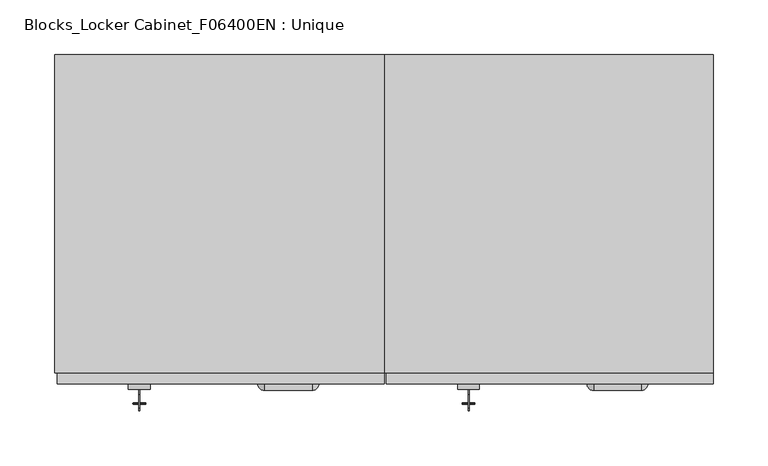
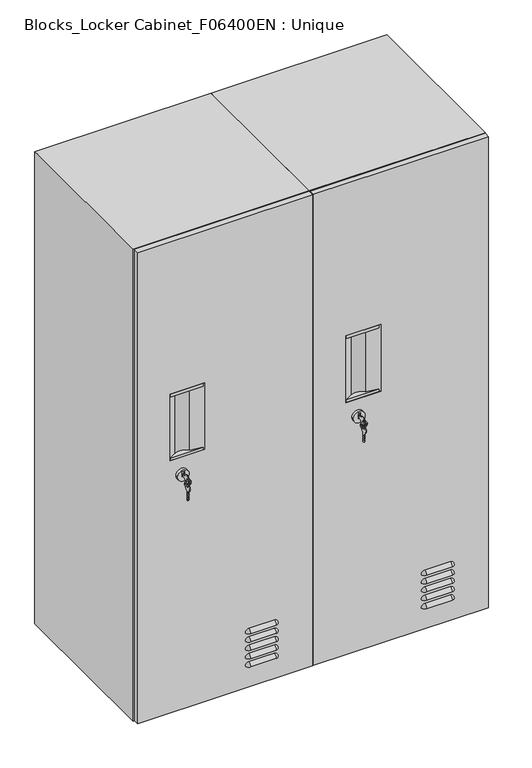
"""IFC4 building model written with IfcOpenShell, lengths in millimetres: furniture geometry, Blocks_Locker Cabinet_F06400EN : Unique."""

from ifc_helpers import new_model, si_unit, point, frame, frame_2d, origin, place, context, project, spatial, polyline, circle_curve, ellipse_curve, trimmed, segment, composite_curve, outline, extrude, faceted_brep, source, transform, mapped, element, save
from ifc_brep_helpers import plane_surface, cylinder_surface, revolved_surface, advanced_brep


def blocks_locker_cabinet_f06400en_unique_ebf76149(model_context):
    return source(origin(), model_context, "Body", "SolidModel", [
        advanced_brep(
        [(-83.0, -12.5, 1375.0), (-63.0, -12.5, 1375.0), (-71.1588195, -12.5, 1382.0962926), (-71.1588195, -12.5, 1372.8618188), (-74.8411805, -12.5, 1372.8618188), (-74.8411805, -12.5, 1382.0962926), (-83.0, -7.5, 1375.0), (-63.0, -7.5, 1375.0), (-83.0, -10.7450625, 1375.0), (-63.0, -10.7450625, 1375.0), (-71.1588195, -10.7450625, 1382.0962926), (-71.1588195, -10.7450625, 1372.8618188), (-74.8411805, -10.7450625, 1372.8618188), (-74.8411805, -10.7450625, 1382.0962926)],
        [
            (0, 1, circle_curve(frame((-73.0, -12.5, 1375.0), z_axis=(0.0, -1.0, 0.0), x_axis=(1.0, 0.0, 0.0)), 10.0)),
            (1, 0, circle_curve(frame((-73.0, -12.5, 1375.0), z_axis=(0.0, -1.0, 0.0), x_axis=(1.0, 0.0, 0.0)), 10.0)),
            (2, 3),
            (3, 4),
            (4, 5),
            (5, 2),
            (6, 7, circle_curve(frame((-73.0, -7.5, 1375.0), z_axis=(0.0, 1.0, 0.0), x_axis=(1.0, 0.0, 0.0)), 10.0)),
            (7, 6, circle_curve(frame((-73.0, -7.5, 1375.0), z_axis=(0.0, 1.0, 0.0), x_axis=(1.0, 0.0, 0.0)), 10.0)),
            (0, 8),
            (8, 6),
            (7, 9),
            (9, 1),
            (2, 10),
            (10, 11),
            (11, 3),
            (11, 12),
            (12, 4),
            (12, 13),
            (13, 5),
            (13, 10),
        ],
        [
            plane_surface(frame((-63.0, -12.5, 1375.0), z_axis=(0.0, -1.0, 0.0), x_axis=(0.0, 0.0, 1.0))),
            plane_surface(frame((-63.0, -7.5, 1375.0), z_axis=(0.0, 1.0, 0.0), x_axis=(0.0, 0.0, -1.0))),
            cylinder_surface(frame((-73.0, -7.5, 1375.0), z_axis=(0.0, -1.0, 0.0), x_axis=(1.0, 0.0, 0.0)), 10.0),
            plane_surface(frame((-71.1588195, -12.5, 1382.0962926), z_axis=(-1.0, 0.0, 0.0), x_axis=(0.0, 1.0, 0.0))),
            plane_surface(frame((-71.1588195, -12.5, 1372.8618188), z_axis=(0.0, 0.0, 1.0), x_axis=(0.0, 1.0, 0.0))),
            plane_surface(frame((-74.8411805, -12.5, 1372.8618188), z_axis=(1.0, 0.0, 0.0), x_axis=(0.0, 1.0, 0.0))),
            plane_surface(frame((-74.8411805, -12.5, 1382.0962926), z_axis=(0.0, 0.0, -1.0), x_axis=(0.0, 1.0, 0.0))),
            plane_surface(frame((-63.0, -10.7450625, 1375.0), z_axis=(0.0, -1.0, 0.0), x_axis=(0.0, 0.0, 1.0))),
        ],
        [
            (0, [[1, 2], [3, 4, 5, 6]]),
            (1, [[7, 8]]),
            (2, [[-1, 9, 10, -8, 11, 12]]),
            (2, [[-2, -12, -11, -7, -10, -9]]),
            (3, [[-3, 13, 14, 15]]),
            (4, [[-4, -15, 16, 17]]),
            (5, [[-5, -17, 18, 19]]),
            (6, [[-6, -19, 20, -13]]),
            (7, [[-14, -20, -18, -16]]),
        ],
    ),
        extrude(outline(composite_curve([segment(trimmed(circle_curve(frame_2d((-23.0067332, 1375.0)), 6.5414185), [point((-16.8246351, 1372.8618188))], [point((-17.0336838, 1377.6669902))], False, "CARTESIAN"), True, "CONTINUOUS"), segment(polyline([(-17.0336838, 1377.6669902), (-10.7450625, 1377.6669902), (-10.7450625, 1372.8618188), (-12.0321832, 1372.8618188)]), True, "CONTINUOUS"), segment(trimmed(circle_curve(frame_2d((-12.908516, 1372.8618188)), 0.8763328), [point((-12.0321832, 1372.8618188))], [point((-13.7848488, 1372.8618188))], True, "CARTESIAN"), True, "CONTINUOUS"), segment(polyline([(-13.7848488, 1372.8618188), (-16.8246351, 1372.8618188)]), True, "CONTINUOUS")], self_intersect=False), holes=[composite_curve([segment(trimmed(circle_curve(frame_2d((-25.6281997, 1375.0)), 1.688217), [point((-27.3164167, 1375.0))], [point((-23.9399827, 1375.0))], True, "CARTESIAN"), True, "CONTINUOUS"), segment(trimmed(circle_curve(frame_2d((-25.6281997, 1375.0)), 1.688217), [point((-23.9399827, 1375.0))], [point((-27.3164167, 1375.0))], True, "CARTESIAN"), True, "CONTINUOUS")], self_intersect=False)]), frame((-73.4043078, 0.0, 0.0), z_axis=(1.0, 0.0, 0.0), x_axis=(0.0, 1.0, 0.0)), (0.0, 0.0, 1.0), 0.9157402),
        extrude(outline(composite_curve([segment(trimmed(circle_curve(frame_2d((-25.6743188, 1360.9839856)), 6.5414185), [point((-27.8125, 1354.8018875))], [point((-24.2573286, 1354.5978839))], False, "CARTESIAN"), True, "CONTINUOUS"), segment(polyline([(-24.2573286, 1354.5978839), (-24.2573286, 1337.7095301), (-25.9613419, 1337.7095301), (-27.8125, 1340.3532579), (-27.8125, 1342.0094356)]), True, "CONTINUOUS"), segment(trimmed(circle_curve(frame_2d((-27.8125, 1342.8857684)), 0.8763328), [point((-27.8125, 1342.0094356))], [point((-27.8125, 1343.7621012))], True, "CARTESIAN"), True, "CONTINUOUS"), segment(polyline([(-27.8125, 1343.7621012), (-27.8125, 1346.0094356)]), True, "CONTINUOUS"), segment(trimmed(circle_curve(frame_2d((-27.8125, 1346.8857684)), 0.8763328), [point((-27.8125, 1346.0094356))], [point((-27.8125, 1347.7621012))], True, "CARTESIAN"), True, "CONTINUOUS"), segment(polyline([(-27.8125, 1347.7621012), (-27.8125, 1350.0094356)]), True, "CONTINUOUS"), segment(trimmed(circle_curve(frame_2d((-27.8125, 1350.8857684)), 0.8763328), [point((-27.8125, 1350.0094356))], [point((-27.8125, 1351.7621012))], True, "CARTESIAN"), True, "CONTINUOUS"), segment(polyline([(-27.8125, 1351.7621012), (-27.8125, 1354.8018875)]), True, "CONTINUOUS")], self_intersect=False), holes=[composite_curve([segment(trimmed(circle_curve(frame_2d((-25.6743188, 1363.6054521)), 1.688217), [point((-25.6743188, 1365.2936691))], [point((-25.6743188, 1361.9172351))], True, "CARTESIAN"), True, "CONTINUOUS"), segment(trimmed(circle_curve(frame_2d((-25.6743188, 1363.6054521)), 1.688217), [point((-25.6743188, 1361.9172351))], [point((-25.6743188, 1365.2936691))], True, "CARTESIAN"), True, "CONTINUOUS")], self_intersect=False)]), frame((-73.4043078, 0.0, 0.0), z_axis=(1.0, 0.0, 0.0), x_axis=(0.0, 1.0, 0.0)), (0.0, 0.0, 1.0), 0.9157402),
        advanced_brep(
        [(-68.8, -25.663019, 1369.4000012), (-77.2, -25.663019, 1369.4000012), (-78.8, -25.663019, 1369.4000012), (-67.2, -25.663019, 1369.4000012)],
        [
            (0, 1, circle_curve(frame((-73.0, -25.663019, 1369.4000012), z_axis=(0.0, 1.0, 0.0), x_axis=(-1.0, 0.0, 0.0)), 4.2)),
            (1, 2, circle_curve(frame((-78.0, -25.663019, 1369.4000012), z_axis=(0.0, 0.0, -1.0), x_axis=(1.0, 0.0, 0.0)), 0.8)),
            (2, 3, circle_curve(frame((-73.0, -25.663019, 1369.4000012), z_axis=(0.0, -1.0, 0.0), x_axis=(-1.0, 0.0, 0.0)), 5.8)),
            (3, 0, circle_curve(frame((-68.0, -25.663019, 1369.4000012), z_axis=(0.0, 0.0, -1.0), x_axis=(-1.0, 0.0, 0.0)), 0.8)),
            (2, 1, circle_curve(frame((-78.0, -25.663019, 1369.4000012), z_axis=(0.0, 0.0, -1.0), x_axis=(1.0, 0.0, 0.0)), 0.8)),
            (0, 3, circle_curve(frame((-68.0, -25.663019, 1369.4000012), z_axis=(0.0, 0.0, -1.0), x_axis=(-1.0, 0.0, 0.0)), 0.8)),
            (1, 0, circle_curve(frame((-73.0, -25.663019, 1369.4000012), z_axis=(0.0, 1.0, 0.0), x_axis=(1.0, 0.0, 0.0)), 4.2)),
            (3, 2, circle_curve(frame((-73.0, -25.663019, 1369.4000012), z_axis=(0.0, -1.0, 0.0), x_axis=(1.0, 0.0, 0.0)), 5.8)),
        ],
        [
            revolved_surface(trimmed(ellipse_curve(frame((-78.0, -25.663019, 1369.4000012), z_axis=(0.0, 0.0, 1.0), x_axis=(1.0, 0.0, 0.0)), 0.8, 0.8), [point((-78.8, -25.663019, 1369.4000012))], [point((-77.2, -25.663019, 1369.4000012))], True, "CARTESIAN"), (-73.0, 2.5, 1369.4000012), (0.0, -1.0, 0.0)),
            revolved_surface(trimmed(ellipse_curve(frame((-78.0, -25.663019, 1369.4000012), z_axis=(0.0, 0.0, 1.0), x_axis=(1.0, 0.0, 0.0)), 0.8, 0.8), [point((-77.2, -25.663019, 1369.4000012))], [point((-78.8, -25.663019, 1369.4000012))], True, "CARTESIAN"), (-73.0, 2.5, 1369.4000012), (0.0, -1.0, 0.0)),
            revolved_surface(trimmed(ellipse_curve(frame((-68.0, -25.663019, 1369.4000012), z_axis=(0.0, 0.0, -1.0), x_axis=(-1.0, 0.0, 0.0)), 0.8, 0.8), [point((-67.2, -25.663019, 1369.4000012))], [point((-68.8, -25.663019, 1369.4000012))], True, "CARTESIAN"), (-73.0, 2.5, 1369.4000012), (0.0, -1.0, 0.0)),
            revolved_surface(trimmed(ellipse_curve(frame((-68.0, -25.663019, 1369.4000012), z_axis=(0.0, 0.0, -1.0), x_axis=(-1.0, 0.0, 0.0)), 0.8, 0.8), [point((-68.8, -25.663019, 1369.4000012))], [point((-67.2, -25.663019, 1369.4000012))], True, "CARTESIAN"), (-73.0, 2.5, 1369.4000012), (0.0, -1.0, 0.0)),
        ],
        [
            (0, [[1, 2, 3, 4]]),
            (1, [[-3, 5, -1, 6]]),
            (2, [[7, -4, 8, -2]]),
            (3, [[-8, -6, -7, -5]]),
        ],
    ),
        advanced_brep(
        [(-148.0, -7.5, 1799.0), (150.0, -7.5, 1799.0), (150.0, 2.5, 1799.0), (-148.0, 2.5, 1799.0), (-148.0, -7.5, 951.0), (-148.0, 2.5, 951.0), (150.0, 2.5, 951.0), (150.0, -7.5, 951.0), (-93.0, -7.5, 1525.0), (-33.7890736, -7.5, 1525.0), (-33.7890736, -7.5, 1405.0), (-93.0, -7.5, 1405.0), (-80.6526901, -0.3712773, 1525.0), (-57.2105549, -3.975278, 1525.0), (-80.6526901, -0.3712773, 1405.0), (-57.2105549, -3.975278, 1405.0)],
        [
            (0, 1),
            (1, 2),
            (2, 3),
            (3, 0),
            (4, 5),
            (5, 6),
            (6, 7),
            (7, 4),
            (0, 4),
            (7, 1),
            (8, 9),
            (9, 10),
            (10, 11),
            (11, 8),
            (6, 2),
            (5, 3),
            (12, 13, circle_curve(frame((-71.1776523, -16.7825242, 1525.0), z_axis=(0.0, 0.0, -1.0), x_axis=(0.0, -1.0, 0.0)), 18.9500756)),
            (13, 9),
            (8, 12),
            (14, 11),
            (10, 15),
            (15, 14, circle_curve(frame((-71.1776523, -16.7825242, 1405.0), z_axis=(0.0, 0.0, 1.0), x_axis=(0.0, -1.0, 0.0)), 18.9500756)),
            (14, 12),
            (13, 15),
        ],
        [
            plane_surface(frame((150.0, -7.5, 1799.0), z_axis=(0.0, 0.0, 1.0), x_axis=(1.0, 0.0, 0.0))),
            plane_surface(frame((150.0, -7.5, 951.0), z_axis=(0.0, 0.0, -1.0), x_axis=(-1.0, 0.0, 0.0))),
            plane_surface(frame((-148.0, -7.5, 1799.0), z_axis=(0.0, -1.0, 0.0), x_axis=(0.0, 0.0, -1.0))),
            plane_surface(frame((150.0, -7.5, 1799.0), z_axis=(1.0, 0.0, 0.0), x_axis=(0.0, 0.0, -1.0))),
            plane_surface(frame((150.0, 2.5, 1799.0), z_axis=(0.0, 1.0, 0.0), x_axis=(0.0, 0.0, -1.0))),
            plane_surface(frame((-148.0, 2.5, 1799.0), z_axis=(-1.0, 0.0, 0.0), x_axis=(0.0, 0.0, -1.0))),
            plane_surface(frame((-93.0, -7.5, 1525.0), z_axis=(0.0, 0.0, -1.0), x_axis=(-0.866025403784437, -0.5000000000000028, 0.0))),
            plane_surface(frame((-93.0, -7.5, 1405.0), z_axis=(0.0, 0.0, 1.0), x_axis=(0.866025403784437, 0.5000000000000028, 0.0))),
            plane_surface(frame((-80.6526901, -0.3712773, 1525.0), z_axis=(0.5000000000000028, -0.866025403784437, 0.0), x_axis=(0.0, 0.0, -1.0))),
            plane_surface(frame((-33.7890736, -7.5, 1525.0), z_axis=(-0.14881527984319862, -0.9888650122666847, 0.0), x_axis=(0.0, 0.0, -1.0))),
            revolved_surface(polyline([(-71.1776523, -35.7325998, 1525.0), (-71.1776523, -35.7325998, 1405.0)]), (-71.1776523, -16.7825242, 1405.0), (0.0, 0.0, 1.0)),
        ],
        [
            (0, [[1, 2, 3, 4]]),
            (1, [[5, 6, 7, 8]]),
            (2, [[-1, 9, -8, 10], [11, 12, 13, 14]]),
            (3, [[-2, -10, -7, 15]]),
            (4, [[-3, -15, -6, 16]]),
            (5, [[-4, -16, -5, -9]]),
            (6, [[17, 18, -11, 19]]),
            (7, [[20, -13, 21, 22]]),
            (8, [[-19, -14, -20, 23]]),
            (9, [[-18, 24, -21, -12]]),
            (10, [[-17, -23, -22, -24]]),
        ],
    ),
        advanced_brep(
        [(35.0, -7.5, 991.0), (41.0, -7.5, 997.0), (84.5189667, -7.5, 997.0), (90.5189667, -7.5, 991.0), (84.5189667, -13.5, 991.0), (41.0, -13.5, 991.0)],
        [
            (0, 1, circle_curve(frame((41.0, -7.5, 991.0), z_axis=(0.0, 1.0, 0.0), x_axis=(1.0, 0.0, 0.0)), 6.0)),
            (1, 2),
            (2, 3, circle_curve(frame((84.5189667, -7.5, 991.0), z_axis=(0.0, 1.0, 0.0), x_axis=(1.0, 0.0, 0.0)), 6.0)),
            (3, 0),
            (3, 4, circle_curve(frame((84.5189667, -7.5, 991.0), z_axis=(0.0, 0.0, -1.0), x_axis=(1.0, 0.0, 0.0)), 6.0)),
            (4, 5),
            (5, 0, circle_curve(frame((41.0, -7.5, 991.0), z_axis=(0.0, 0.0, -1.0), x_axis=(1.0, 0.0, 0.0)), 6.0)),
            (5, 1, circle_curve(frame((41.0, -7.5, 991.0), z_axis=(-1.0, 0.0, 0.0), x_axis=(0.0, 0.0, 1.0)), 6.0)),
            (4, 2, circle_curve(frame((84.5189667, -7.5, 991.0), z_axis=(-1.0, 0.0, 0.0), x_axis=(0.0, 0.0, 1.0)), 6.0)),
        ],
        [
            plane_surface(frame((85.0, -7.5, 991.0), z_axis=(0.0, 1.0, 0.0), x_axis=(0.0, 0.0, 1.0))),
            plane_surface(frame((85.0, -7.5, 991.0), z_axis=(0.0, 0.0, -1.0), x_axis=(0.0, -1.0, 0.0))),
            revolved_surface(trimmed(ellipse_curve(frame((41.0, -7.5, 991.0), z_axis=(0.0, 1.0, 0.0), x_axis=(1.0, 0.0, 0.0)), 6.0, 6.0), [point((35.0, -7.5, 991.0))], [point((41.0, -7.5, 997.0))], True, "CARTESIAN"), (85.0, -7.5, 991.0), (1.0, 0.0, 0.0)),
            cylinder_surface(frame((85.0, -7.5, 991.0), z_axis=(1.0, 0.0, 0.0), x_axis=(0.0, 0.0, 1.0)), 6.0),
            revolved_surface(trimmed(ellipse_curve(frame((84.5189667, -7.5, 991.0), z_axis=(0.0, 1.0, 0.0), x_axis=(1.0, 0.0, 0.0)), 6.0, 6.0), [point((84.5189667, -7.5, 997.0))], [point((90.5189667, -7.5, 991.0))], True, "CARTESIAN"), (85.0, -7.5, 991.0), (1.0, 0.0, 0.0)),
        ],
        [
            (0, [[1, 2, 3, 4]]),
            (1, [[5, 6, 7, -4]]),
            (2, [[8, -1, -7]]),
            (3, [[9, -2, -8, -6]]),
            (4, [[-3, -9, -5]]),
        ],
    ),
        advanced_brep(
        [(35.0, -7.5, 1006.0), (41.0, -7.5, 1012.0), (84.5189667, -7.5, 1012.0), (90.5189667, -7.5, 1006.0), (84.5189667, -13.5, 1006.0), (41.0, -13.5, 1006.0)],
        [
            (0, 1, circle_curve(frame((41.0, -7.5, 1006.0), z_axis=(0.0, 1.0, 0.0), x_axis=(1.0, 0.0, 0.0)), 6.0)),
            (1, 2),
            (2, 3, circle_curve(frame((84.5189667, -7.5, 1006.0), z_axis=(0.0, 1.0, 0.0), x_axis=(1.0, 0.0, 0.0)), 6.0)),
            (3, 0),
            (3, 4, circle_curve(frame((84.5189667, -7.5, 1006.0), z_axis=(0.0, 0.0, -1.0), x_axis=(1.0, 0.0, 0.0)), 6.0)),
            (4, 5),
            (5, 0, circle_curve(frame((41.0, -7.5, 1006.0), z_axis=(0.0, 0.0, -1.0), x_axis=(1.0, 0.0, 0.0)), 6.0)),
            (5, 1, circle_curve(frame((41.0, -7.5, 1006.0), z_axis=(-1.0, 0.0, 0.0), x_axis=(0.0, 0.0, 1.0)), 6.0)),
            (4, 2, circle_curve(frame((84.5189667, -7.5, 1006.0), z_axis=(-1.0, 0.0, 0.0), x_axis=(0.0, 0.0, 1.0)), 6.0)),
        ],
        [
            plane_surface(frame((85.0, -7.5, 1006.0), z_axis=(0.0, 1.0, 0.0), x_axis=(0.0, 0.0, 1.0))),
            plane_surface(frame((85.0, -7.5, 1006.0), z_axis=(0.0, 0.0, -1.0), x_axis=(0.0, -1.0, 0.0))),
            revolved_surface(trimmed(ellipse_curve(frame((41.0, -7.5, 1006.0), z_axis=(0.0, 1.0, 0.0), x_axis=(1.0, 0.0, 0.0)), 6.0, 6.0), [point((35.0, -7.5, 1006.0))], [point((41.0, -7.5, 1012.0))], True, "CARTESIAN"), (85.0, -7.5, 1006.0), (1.0, 0.0, 0.0)),
            cylinder_surface(frame((85.0, -7.5, 1006.0), z_axis=(1.0, 0.0, 0.0), x_axis=(0.0, 0.0, 1.0)), 6.0),
            revolved_surface(trimmed(ellipse_curve(frame((84.5189667, -7.5, 1006.0), z_axis=(0.0, 1.0, 0.0), x_axis=(1.0, 0.0, 0.0)), 6.0, 6.0), [point((84.5189667, -7.5, 1012.0))], [point((90.5189667, -7.5, 1006.0))], True, "CARTESIAN"), (85.0, -7.5, 1006.0), (1.0, 0.0, 0.0)),
        ],
        [
            (0, [[1, 2, 3, 4]]),
            (1, [[5, 6, 7, -4]]),
            (2, [[8, -1, -7]]),
            (3, [[9, -2, -8, -6]]),
            (4, [[-3, -9, -5]]),
        ],
    ),
        advanced_brep(
        [(35.0, -7.5, 1021.0), (41.0, -7.5, 1027.0), (84.5189667, -7.5, 1027.0), (90.5189667, -7.5, 1021.0), (84.5189667, -13.5, 1021.0), (41.0, -13.5, 1021.0)],
        [
            (0, 1, circle_curve(frame((41.0, -7.5, 1021.0), z_axis=(0.0, 1.0, 0.0), x_axis=(1.0, 0.0, 0.0)), 6.0)),
            (1, 2),
            (2, 3, circle_curve(frame((84.5189667, -7.5, 1021.0), z_axis=(0.0, 1.0, 0.0), x_axis=(1.0, 0.0, 0.0)), 6.0)),
            (3, 0),
            (3, 4, circle_curve(frame((84.5189667, -7.5, 1021.0), z_axis=(0.0, 0.0, -1.0), x_axis=(1.0, 0.0, 0.0)), 6.0)),
            (4, 5),
            (5, 0, circle_curve(frame((41.0, -7.5, 1021.0), z_axis=(0.0, 0.0, -1.0), x_axis=(1.0, 0.0, 0.0)), 6.0)),
            (5, 1, circle_curve(frame((41.0, -7.5, 1021.0), z_axis=(-1.0, 0.0, 0.0), x_axis=(0.0, 0.0, 1.0)), 6.0)),
            (4, 2, circle_curve(frame((84.5189667, -7.5, 1021.0), z_axis=(-1.0, 0.0, 0.0), x_axis=(0.0, 0.0, 1.0)), 6.0)),
        ],
        [
            plane_surface(frame((85.0, -7.5, 1021.0), z_axis=(0.0, 1.0, 0.0), x_axis=(0.0, 0.0, 1.0))),
            plane_surface(frame((85.0, -7.5, 1021.0), z_axis=(0.0, 0.0, -1.0), x_axis=(0.0, -1.0, 0.0))),
            revolved_surface(trimmed(ellipse_curve(frame((41.0, -7.5, 1021.0), z_axis=(0.0, 1.0, 0.0), x_axis=(1.0, 0.0, 0.0)), 6.0, 6.0), [point((35.0, -7.5, 1021.0))], [point((41.0, -7.5, 1027.0))], True, "CARTESIAN"), (85.0, -7.5, 1021.0), (1.0, 0.0, 0.0)),
            cylinder_surface(frame((85.0, -7.5, 1021.0), z_axis=(1.0, 0.0, 0.0), x_axis=(0.0, 0.0, 1.0)), 6.0),
            revolved_surface(trimmed(ellipse_curve(frame((84.5189667, -7.5, 1021.0), z_axis=(0.0, 1.0, 0.0), x_axis=(1.0, 0.0, 0.0)), 6.0, 6.0), [point((84.5189667, -7.5, 1027.0))], [point((90.5189667, -7.5, 1021.0))], True, "CARTESIAN"), (85.0, -7.5, 1021.0), (1.0, 0.0, 0.0)),
        ],
        [
            (0, [[1, 2, 3, 4]]),
            (1, [[5, 6, 7, -4]]),
            (2, [[8, -1, -7]]),
            (3, [[9, -2, -8, -6]]),
            (4, [[-3, -9, -5]]),
        ],
    ),
        advanced_brep(
        [(35.0, -7.5, 1036.0), (41.0, -7.5, 1042.0), (84.5189667, -7.5, 1042.0), (90.5189667, -7.5, 1036.0), (84.5189667, -13.5, 1036.0), (41.0, -13.5, 1036.0)],
        [
            (0, 1, circle_curve(frame((41.0, -7.5, 1036.0), z_axis=(0.0, 1.0, 0.0), x_axis=(1.0, 0.0, 0.0)), 6.0)),
            (1, 2),
            (2, 3, circle_curve(frame((84.5189667, -7.5, 1036.0), z_axis=(0.0, 1.0, 0.0), x_axis=(1.0, 0.0, 0.0)), 6.0)),
            (3, 0),
            (3, 4, circle_curve(frame((84.5189667, -7.5, 1036.0), z_axis=(0.0, 0.0, -1.0), x_axis=(1.0, 0.0, 0.0)), 6.0)),
            (4, 5),
            (5, 0, circle_curve(frame((41.0, -7.5, 1036.0), z_axis=(0.0, 0.0, -1.0), x_axis=(1.0, 0.0, 0.0)), 6.0)),
            (5, 1, circle_curve(frame((41.0, -7.5, 1036.0), z_axis=(-1.0, 0.0, 0.0), x_axis=(0.0, 0.0, 1.0)), 6.0)),
            (4, 2, circle_curve(frame((84.5189667, -7.5, 1036.0), z_axis=(-1.0, 0.0, 0.0), x_axis=(0.0, 0.0, 1.0)), 6.0)),
        ],
        [
            plane_surface(frame((85.0, -7.5, 1036.0), z_axis=(0.0, 1.0, 0.0), x_axis=(0.0, 0.0, 1.0))),
            plane_surface(frame((85.0, -7.5, 1036.0), z_axis=(0.0, 0.0, -1.0), x_axis=(0.0, -1.0, 0.0))),
            revolved_surface(trimmed(ellipse_curve(frame((41.0, -7.5, 1036.0), z_axis=(0.0, 1.0, 0.0), x_axis=(1.0, 0.0, 0.0)), 6.0, 6.0), [point((35.0, -7.5, 1036.0))], [point((41.0, -7.5, 1042.0))], True, "CARTESIAN"), (85.0, -7.5, 1036.0), (1.0, 0.0, 0.0)),
            cylinder_surface(frame((85.0, -7.5, 1036.0), z_axis=(1.0, 0.0, 0.0), x_axis=(0.0, 0.0, 1.0)), 6.0),
            revolved_surface(trimmed(ellipse_curve(frame((84.5189667, -7.5, 1036.0), z_axis=(0.0, 1.0, 0.0), x_axis=(1.0, 0.0, 0.0)), 6.0, 6.0), [point((84.5189667, -7.5, 1042.0))], [point((90.5189667, -7.5, 1036.0))], True, "CARTESIAN"), (85.0, -7.5, 1036.0), (1.0, 0.0, 0.0)),
        ],
        [
            (0, [[1, 2, 3, 4]]),
            (1, [[5, 6, 7, -4]]),
            (2, [[8, -1, -7]]),
            (3, [[9, -2, -8, -6]]),
            (4, [[-3, -9, -5]]),
        ],
    ),
        advanced_brep(
        [(35.0, -7.5, 1051.0), (41.0, -7.5, 1057.0), (84.5189667, -7.5, 1057.0), (90.5189667, -7.5, 1051.0), (84.5189667, -13.5, 1051.0), (41.0, -13.5, 1051.0)],
        [
            (0, 1, circle_curve(frame((41.0, -7.5, 1051.0), z_axis=(0.0, 1.0, 0.0), x_axis=(1.0, 0.0, 0.0)), 6.0)),
            (1, 2),
            (2, 3, circle_curve(frame((84.5189667, -7.5, 1051.0), z_axis=(0.0, 1.0, 0.0), x_axis=(1.0, 0.0, 0.0)), 6.0)),
            (3, 0),
            (3, 4, circle_curve(frame((84.5189667, -7.5, 1051.0), z_axis=(0.0, 0.0, -1.0), x_axis=(1.0, 0.0, 0.0)), 6.0)),
            (4, 5),
            (5, 0, circle_curve(frame((41.0, -7.5, 1051.0), z_axis=(0.0, 0.0, -1.0), x_axis=(1.0, 0.0, 0.0)), 6.0)),
            (5, 1, circle_curve(frame((41.0, -7.5, 1051.0), z_axis=(-1.0, 0.0, 0.0), x_axis=(0.0, 0.0, 1.0)), 6.0)),
            (4, 2, circle_curve(frame((84.5189667, -7.5, 1051.0), z_axis=(-1.0, 0.0, 0.0), x_axis=(0.0, 0.0, 1.0)), 6.0)),
        ],
        [
            plane_surface(frame((85.0, -7.5, 1051.0), z_axis=(0.0, 1.0, 0.0), x_axis=(0.0, 0.0, 1.0))),
            plane_surface(frame((85.0, -7.5, 1051.0), z_axis=(0.0, 0.0, -1.0), x_axis=(0.0, -1.0, 0.0))),
            revolved_surface(trimmed(ellipse_curve(frame((41.0, -7.5, 1051.0), z_axis=(0.0, 1.0, 0.0), x_axis=(1.0, 0.0, 0.0)), 6.0, 6.0), [point((35.0, -7.5, 1051.0))], [point((41.0, -7.5, 1057.0))], True, "CARTESIAN"), (85.0, -7.5, 1051.0), (1.0, 0.0, 0.0)),
            cylinder_surface(frame((85.0, -7.5, 1051.0), z_axis=(1.0, 0.0, 0.0), x_axis=(0.0, 0.0, 1.0)), 6.0),
            revolved_surface(trimmed(ellipse_curve(frame((84.5189667, -7.5, 1051.0), z_axis=(0.0, 1.0, 0.0), x_axis=(1.0, 0.0, 0.0)), 6.0, 6.0), [point((84.5189667, -7.5, 1057.0))], [point((90.5189667, -7.5, 1051.0))], True, "CARTESIAN"), (85.0, -7.5, 1051.0), (1.0, 0.0, 0.0)),
        ],
        [
            (0, [[1, 2, 3, 4]]),
            (1, [[5, 6, 7, -4]]),
            (2, [[8, -1, -7]]),
            (3, [[9, -2, -8, -6]]),
            (4, [[-3, -9, -5]]),
        ],
    ),
        extrude(outline(composite_curve([segment(trimmed(circle_curve(frame_2d((-71.1776523, -16.7825242)), 18.9500756), [point((-80.6526901, -0.3712773))], [point((-57.2105549, -3.975278))], False, "CARTESIAN"), True, "CONTINUOUS"), segment(polyline([(-57.2105549, -3.975278), (-33.7890736, -7.5), (-93.0, -7.5), (-80.6526901, -0.3712773)]), True, "CONTINUOUS")], self_intersect=False)), frame((0.0, 0.0, 1405.0), z_axis=(0.0, 0.0, 1.0), x_axis=(1.0, 0.0, 0.0)), (0.0, 0.0, 1.0), 5.0),
        extrude(outline(composite_curve([segment(trimmed(circle_curve(frame_2d((-71.1776523, -16.7825242)), 18.9500756), [point((-80.6526901, -0.3712773))], [point((-57.2105549, -3.975278))], False, "CARTESIAN"), True, "CONTINUOUS"), segment(polyline([(-57.2105549, -3.975278), (-33.7890736, -7.5), (-93.0, -7.5), (-80.6526901, -0.3712773)]), True, "CONTINUOUS")], self_intersect=False)), frame((0.0, 0.0, 1520.0), z_axis=(0.0, 0.0, 1.0), x_axis=(1.0, 0.0, 0.0)), (0.0, 0.0, 1.0), 5.0),
        faceted_brep([(150.0, 2.5, 1800.0), (-150.0, 2.5, 1800.0), (-150.0, 2.5, 950.0), (150.0, 2.5, 950.0), (140.0, 2.5, 1790.0), (140.0, 2.5, 960.0), (-140.0, 2.5, 960.0), (-140.0, 2.5, 1790.0), (150.0, 292.5, 1800.0), (150.0, 292.5, 950.0), (-150.0, 292.5, 950.0), (-150.0, 292.5, 1800.0), (150.0, 282.5, 1800.0), (-150.0, 282.5, 1800.0), (-150.0, 282.5, 950.0), (150.0, 282.5, 950.0), (140.0, 282.5, 1790.0), (140.0, 282.5, 960.0), (-140.0, 282.5, 960.0), (-140.0, 282.5, 1790.0)], [[[0, 1, 2, 3], [4, 5, 6, 7]], [[8, 9, 10, 11]], [[1, 0, 12, 8, 11, 13]], [[2, 1, 13, 11, 10, 14]], [[3, 2, 14, 10, 9, 15]], [[0, 3, 15, 9, 8, 12]], [[5, 4, 16, 17]], [[6, 5, 17, 18]], [[7, 6, 18, 19]], [[4, 7, 19, 16]], [[17, 16, 19, 18]]]),
        advanced_brep(
        [(217.0, -12.5, 1375.0), (237.0, -12.5, 1375.0), (228.8411805, -12.5, 1382.0962926), (228.8411805, -12.5, 1372.8618188), (225.1588195, -12.5, 1372.8618188), (225.1588195, -12.5, 1382.0962926), (217.0, -7.5, 1375.0), (237.0, -7.5, 1375.0), (217.0, -10.7450625, 1375.0), (237.0, -10.7450625, 1375.0), (228.8411805, -10.7450625, 1382.0962926), (228.8411805, -10.7450625, 1372.8618188), (225.1588195, -10.7450625, 1372.8618188), (225.1588195, -10.7450625, 1382.0962926)],
        [
            (0, 1, circle_curve(frame((227.0, -12.5, 1375.0), z_axis=(0.0, -1.0, 0.0), x_axis=(1.0, 0.0, 0.0)), 10.0)),
            (1, 0, circle_curve(frame((227.0, -12.5, 1375.0), z_axis=(0.0, -1.0, 0.0), x_axis=(1.0, 0.0, 0.0)), 10.0)),
            (2, 3),
            (3, 4),
            (4, 5),
            (5, 2),
            (6, 7, circle_curve(frame((227.0, -7.5, 1375.0), z_axis=(0.0, 1.0, 0.0), x_axis=(1.0, 0.0, 0.0)), 10.0)),
            (7, 6, circle_curve(frame((227.0, -7.5, 1375.0), z_axis=(0.0, 1.0, 0.0), x_axis=(1.0, 0.0, 0.0)), 10.0)),
            (0, 8),
            (8, 6),
            (7, 9),
            (9, 1),
            (2, 10),
            (10, 11),
            (11, 3),
            (11, 12),
            (12, 4),
            (12, 13),
            (13, 5),
            (13, 10),
        ],
        [
            plane_surface(frame((237.0, -12.5, 1375.0), z_axis=(0.0, -1.0, 0.0), x_axis=(0.0, 0.0, 1.0))),
            plane_surface(frame((237.0, -7.5, 1375.0), z_axis=(0.0, 1.0, 0.0), x_axis=(0.0, 0.0, -1.0))),
            cylinder_surface(frame((227.0, -7.5, 1375.0), z_axis=(0.0, -1.0, 0.0), x_axis=(1.0, 0.0, 0.0)), 10.0),
            plane_surface(frame((228.8411805, -12.5, 1382.0962926), z_axis=(-1.0, 0.0, 0.0), x_axis=(0.0, 1.0, 0.0))),
            plane_surface(frame((228.8411805, -12.5, 1372.8618188), z_axis=(0.0, 0.0, 1.0), x_axis=(0.0, 1.0, 0.0))),
            plane_surface(frame((225.1588195, -12.5, 1372.8618188), z_axis=(1.0, 0.0, 0.0), x_axis=(0.0, 1.0, 0.0))),
            plane_surface(frame((225.1588195, -12.5, 1382.0962926), z_axis=(0.0, 0.0, -1.0), x_axis=(0.0, 1.0, 0.0))),
            plane_surface(frame((237.0, -10.7450625, 1375.0), z_axis=(0.0, -1.0, 0.0), x_axis=(0.0, 0.0, 1.0))),
        ],
        [
            (0, [[1, 2], [3, 4, 5, 6]]),
            (1, [[7, 8]]),
            (2, [[-1, 9, 10, -8, 11, 12]]),
            (2, [[-2, -12, -11, -7, -10, -9]]),
            (3, [[-3, 13, 14, 15]]),
            (4, [[-4, -15, 16, 17]]),
            (5, [[-5, -17, 18, 19]]),
            (6, [[-6, -19, 20, -13]]),
            (7, [[-14, -20, -18, -16]]),
        ],
    ),
        extrude(outline(composite_curve([segment(trimmed(circle_curve(frame_2d((-23.0067332, 1375.0)), 6.5414185), [point((-16.8246351, 1372.8618188))], [point((-17.0336838, 1377.6669902))], False, "CARTESIAN"), True, "CONTINUOUS"), segment(polyline([(-17.0336838, 1377.6669902), (-10.7450625, 1377.6669902), (-10.7450625, 1372.8618188), (-12.0321832, 1372.8618188)]), True, "CONTINUOUS"), segment(trimmed(circle_curve(frame_2d((-12.908516, 1372.8618188)), 0.8763328), [point((-12.0321832, 1372.8618188))], [point((-13.7848488, 1372.8618188))], True, "CARTESIAN"), True, "CONTINUOUS"), segment(polyline([(-13.7848488, 1372.8618188), (-16.8246351, 1372.8618188)]), True, "CONTINUOUS")], self_intersect=False), holes=[composite_curve([segment(trimmed(circle_curve(frame_2d((-25.6281997, 1375.0)), 1.688217), [point((-27.3164167, 1375.0))], [point((-23.9399827, 1375.0))], True, "CARTESIAN"), True, "CONTINUOUS"), segment(trimmed(circle_curve(frame_2d((-25.6281997, 1375.0)), 1.688217), [point((-23.9399827, 1375.0))], [point((-27.3164167, 1375.0))], True, "CARTESIAN"), True, "CONTINUOUS")], self_intersect=False)]), frame((226.5956922, 0.0, 0.0), z_axis=(1.0, 0.0, 0.0), x_axis=(0.0, 1.0, 0.0)), (0.0, 0.0, 1.0), 0.9157402),
        extrude(outline(composite_curve([segment(trimmed(circle_curve(frame_2d((-25.6743188, 1360.9839856)), 6.5414185), [point((-27.8125, 1354.8018875))], [point((-24.2573286, 1354.5978839))], False, "CARTESIAN"), True, "CONTINUOUS"), segment(polyline([(-24.2573286, 1354.5978839), (-24.2573286, 1337.7095301), (-25.9613419, 1337.7095301), (-27.8125, 1340.3532579), (-27.8125, 1342.0094356)]), True, "CONTINUOUS"), segment(trimmed(circle_curve(frame_2d((-27.8125, 1342.8857684)), 0.8763328), [point((-27.8125, 1342.0094356))], [point((-27.8125, 1343.7621012))], True, "CARTESIAN"), True, "CONTINUOUS"), segment(polyline([(-27.8125, 1343.7621012), (-27.8125, 1346.0094356)]), True, "CONTINUOUS"), segment(trimmed(circle_curve(frame_2d((-27.8125, 1346.8857684)), 0.8763328), [point((-27.8125, 1346.0094356))], [point((-27.8125, 1347.7621012))], True, "CARTESIAN"), True, "CONTINUOUS"), segment(polyline([(-27.8125, 1347.7621012), (-27.8125, 1350.0094356)]), True, "CONTINUOUS"), segment(trimmed(circle_curve(frame_2d((-27.8125, 1350.8857684)), 0.8763328), [point((-27.8125, 1350.0094356))], [point((-27.8125, 1351.7621012))], True, "CARTESIAN"), True, "CONTINUOUS"), segment(polyline([(-27.8125, 1351.7621012), (-27.8125, 1354.8018875)]), True, "CONTINUOUS")], self_intersect=False), holes=[composite_curve([segment(trimmed(circle_curve(frame_2d((-25.6743188, 1363.6054521)), 1.688217), [point((-25.6743188, 1365.2936691))], [point((-25.6743188, 1361.9172351))], True, "CARTESIAN"), True, "CONTINUOUS"), segment(trimmed(circle_curve(frame_2d((-25.6743188, 1363.6054521)), 1.688217), [point((-25.6743188, 1361.9172351))], [point((-25.6743188, 1365.2936691))], True, "CARTESIAN"), True, "CONTINUOUS")], self_intersect=False)]), frame((226.5956922, 0.0, 0.0), z_axis=(1.0, 0.0, 0.0), x_axis=(0.0, 1.0, 0.0)), (0.0, 0.0, 1.0), 0.9157402),
        advanced_brep(
        [(231.2, -25.663019, 1369.4000012), (222.8, -25.663019, 1369.4000012), (221.2, -25.663019, 1369.4000012), (232.8, -25.663019, 1369.4000012)],
        [
            (0, 1, circle_curve(frame((227.0, -25.663019, 1369.4000012), z_axis=(0.0, 1.0, 0.0), x_axis=(-1.0, 0.0, 0.0)), 4.2)),
            (1, 2, circle_curve(frame((222.0, -25.663019, 1369.4000012), z_axis=(0.0, 0.0, -1.0), x_axis=(1.0, 0.0, 0.0)), 0.8)),
            (2, 3, circle_curve(frame((227.0, -25.663019, 1369.4000012), z_axis=(0.0, -1.0, 0.0), x_axis=(-1.0, 0.0, 0.0)), 5.8)),
            (3, 0, circle_curve(frame((232.0, -25.663019, 1369.4000012), z_axis=(0.0, 0.0, -1.0), x_axis=(-1.0, 0.0, 0.0)), 0.8)),
            (2, 1, circle_curve(frame((222.0, -25.663019, 1369.4000012), z_axis=(0.0, 0.0, -1.0), x_axis=(1.0, 0.0, 0.0)), 0.8)),
            (0, 3, circle_curve(frame((232.0, -25.663019, 1369.4000012), z_axis=(0.0, 0.0, -1.0), x_axis=(-1.0, 0.0, 0.0)), 0.8)),
            (1, 0, circle_curve(frame((227.0, -25.663019, 1369.4000012), z_axis=(0.0, 1.0, 0.0), x_axis=(1.0, 0.0, 0.0)), 4.2)),
            (3, 2, circle_curve(frame((227.0, -25.663019, 1369.4000012), z_axis=(0.0, -1.0, 0.0), x_axis=(1.0, 0.0, 0.0)), 5.8)),
        ],
        [
            revolved_surface(trimmed(ellipse_curve(frame((222.0, -25.663019, 1369.4000012), z_axis=(0.0, 0.0, 1.0), x_axis=(1.0, 0.0, 0.0)), 0.8, 0.8), [point((221.2, -25.663019, 1369.4000012))], [point((222.8, -25.663019, 1369.4000012))], True, "CARTESIAN"), (227.0, 2.5, 1369.4000012), (0.0, -1.0, 0.0)),
            revolved_surface(trimmed(ellipse_curve(frame((222.0, -25.663019, 1369.4000012), z_axis=(0.0, 0.0, 1.0), x_axis=(1.0, 0.0, 0.0)), 0.8, 0.8), [point((222.8, -25.663019, 1369.4000012))], [point((221.2, -25.663019, 1369.4000012))], True, "CARTESIAN"), (227.0, 2.5, 1369.4000012), (0.0, -1.0, 0.0)),
            revolved_surface(trimmed(ellipse_curve(frame((232.0, -25.663019, 1369.4000012), z_axis=(0.0, 0.0, -1.0), x_axis=(-1.0, 0.0, 0.0)), 0.8, 0.8), [point((232.8, -25.663019, 1369.4000012))], [point((231.2, -25.663019, 1369.4000012))], True, "CARTESIAN"), (227.0, 2.5, 1369.4000012), (0.0, -1.0, 0.0)),
            revolved_surface(trimmed(ellipse_curve(frame((232.0, -25.663019, 1369.4000012), z_axis=(0.0, 0.0, -1.0), x_axis=(-1.0, 0.0, 0.0)), 0.8, 0.8), [point((231.2, -25.663019, 1369.4000012))], [point((232.8, -25.663019, 1369.4000012))], True, "CARTESIAN"), (227.0, 2.5, 1369.4000012), (0.0, -1.0, 0.0)),
        ],
        [
            (0, [[1, 2, 3, 4]]),
            (1, [[-3, 5, -1, 6]]),
            (2, [[7, -4, 8, -2]]),
            (3, [[-8, -6, -7, -5]]),
        ],
    ),
        advanced_brep(
        [(152.0, -7.5, 1799.0), (450.0, -7.5, 1799.0), (450.0, 2.5, 1799.0), (152.0, 2.5, 1799.0), (152.0, -7.5, 951.0), (152.0, 2.5, 951.0), (450.0, 2.5, 951.0), (450.0, -7.5, 951.0), (207.0, -7.5, 1525.0), (266.2109264, -7.5, 1525.0), (266.2109264, -7.5, 1405.0), (207.0, -7.5, 1405.0), (219.3473099, -0.3712773, 1525.0), (242.7894451, -3.975278, 1525.0), (219.3473099, -0.3712773, 1405.0), (242.7894451, -3.975278, 1405.0)],
        [
            (0, 1),
            (1, 2),
            (2, 3),
            (3, 0),
            (4, 5),
            (5, 6),
            (6, 7),
            (7, 4),
            (0, 4),
            (7, 1),
            (8, 9),
            (9, 10),
            (10, 11),
            (11, 8),
            (6, 2),
            (5, 3),
            (12, 13, circle_curve(frame((228.8223477, -16.7825242, 1525.0), z_axis=(0.0, 0.0, -1.0), x_axis=(0.0, -1.0, 0.0)), 18.9500756)),
            (13, 9),
            (8, 12),
            (14, 11),
            (10, 15),
            (15, 14, circle_curve(frame((228.8223477, -16.7825242, 1405.0), z_axis=(0.0, 0.0, 1.0), x_axis=(0.0, -1.0, 0.0)), 18.9500756)),
            (14, 12),
            (13, 15),
        ],
        [
            plane_surface(frame((450.0, -7.5, 1799.0), z_axis=(0.0, 0.0, 1.0), x_axis=(1.0, 0.0, 0.0))),
            plane_surface(frame((450.0, -7.5, 951.0), z_axis=(0.0, 0.0, -1.0), x_axis=(-1.0, 0.0, 0.0))),
            plane_surface(frame((152.0, -7.5, 1799.0), z_axis=(0.0, -1.0, 0.0), x_axis=(0.0, 0.0, -1.0))),
            plane_surface(frame((450.0, -7.5, 1799.0), z_axis=(1.0, 0.0, 0.0), x_axis=(0.0, 0.0, -1.0))),
            plane_surface(frame((450.0, 2.5, 1799.0), z_axis=(0.0, 1.0, 0.0), x_axis=(0.0, 0.0, -1.0))),
            plane_surface(frame((152.0, 2.5, 1799.0), z_axis=(-1.0, 0.0, 0.0), x_axis=(0.0, 0.0, -1.0))),
            plane_surface(frame((207.0, -7.5, 1525.0), z_axis=(0.0, 0.0, -1.0), x_axis=(-0.866025403784437, -0.5000000000000028, 0.0))),
            plane_surface(frame((207.0, -7.5, 1405.0), z_axis=(0.0, 0.0, 1.0), x_axis=(0.866025403784437, 0.5000000000000028, 0.0))),
            plane_surface(frame((219.3473099, -0.3712773, 1525.0), z_axis=(0.5000000000000028, -0.866025403784437, 0.0), x_axis=(0.0, 0.0, -1.0))),
            plane_surface(frame((266.2109264, -7.5, 1525.0), z_axis=(-0.14881527984319862, -0.9888650122666847, 0.0), x_axis=(0.0, 0.0, -1.0))),
            revolved_surface(polyline([(228.8223477, -35.7325998, 1525.0), (228.8223477, -35.7325998, 1405.0)]), (228.8223477, -16.7825242, 1405.0), (0.0, 0.0, 1.0)),
        ],
        [
            (0, [[1, 2, 3, 4]]),
            (1, [[5, 6, 7, 8]]),
            (2, [[-1, 9, -8, 10], [11, 12, 13, 14]]),
            (3, [[-2, -10, -7, 15]]),
            (4, [[-3, -15, -6, 16]]),
            (5, [[-4, -16, -5, -9]]),
            (6, [[17, 18, -11, 19]]),
            (7, [[20, -13, 21, 22]]),
            (8, [[-19, -14, -20, 23]]),
            (9, [[-18, 24, -21, -12]]),
            (10, [[-17, -23, -22, -24]]),
        ],
    ),
        advanced_brep(
        [(335.0, -7.5, 991.0), (341.0, -7.5, 997.0), (384.5189667, -7.5, 997.0), (390.5189667, -7.5, 991.0), (384.5189667, -13.5, 991.0), (341.0, -13.5, 991.0)],
        [
            (0, 1, circle_curve(frame((341.0, -7.5, 991.0), z_axis=(0.0, 1.0, 0.0), x_axis=(1.0, 0.0, 0.0)), 6.0)),
            (1, 2),
            (2, 3, circle_curve(frame((384.5189667, -7.5, 991.0), z_axis=(0.0, 1.0, 0.0), x_axis=(1.0, 0.0, 0.0)), 6.0)),
            (3, 0),
            (3, 4, circle_curve(frame((384.5189667, -7.5, 991.0), z_axis=(0.0, 0.0, -1.0), x_axis=(1.0, 0.0, 0.0)), 6.0)),
            (4, 5),
            (5, 0, circle_curve(frame((341.0, -7.5, 991.0), z_axis=(0.0, 0.0, -1.0), x_axis=(1.0, 0.0, 0.0)), 6.0)),
            (5, 1, circle_curve(frame((341.0, -7.5, 991.0), z_axis=(-1.0, 0.0, 0.0), x_axis=(0.0, 0.0, 1.0)), 6.0)),
            (4, 2, circle_curve(frame((384.5189667, -7.5, 991.0), z_axis=(-1.0, 0.0, 0.0), x_axis=(0.0, 0.0, 1.0)), 6.0)),
        ],
        [
            plane_surface(frame((385.0, -7.5, 991.0), z_axis=(0.0, 1.0, 0.0), x_axis=(0.0, 0.0, 1.0))),
            plane_surface(frame((385.0, -7.5, 991.0), z_axis=(0.0, 0.0, -1.0), x_axis=(0.0, -1.0, 0.0))),
            revolved_surface(trimmed(ellipse_curve(frame((341.0, -7.5, 991.0), z_axis=(0.0, 1.0, 0.0), x_axis=(1.0, 0.0, 0.0)), 6.0, 6.0), [point((335.0, -7.5, 991.0))], [point((341.0, -7.5, 997.0))], True, "CARTESIAN"), (385.0, -7.5, 991.0), (1.0, 0.0, 0.0)),
            cylinder_surface(frame((385.0, -7.5, 991.0), z_axis=(1.0, 0.0, 0.0), x_axis=(0.0, 0.0, 1.0)), 6.0),
            revolved_surface(trimmed(ellipse_curve(frame((384.5189667, -7.5, 991.0), z_axis=(0.0, 1.0, 0.0), x_axis=(1.0, 0.0, 0.0)), 6.0, 6.0), [point((384.5189667, -7.5, 997.0))], [point((390.5189667, -7.5, 991.0))], True, "CARTESIAN"), (385.0, -7.5, 991.0), (1.0, 0.0, 0.0)),
        ],
        [
            (0, [[1, 2, 3, 4]]),
            (1, [[5, 6, 7, -4]]),
            (2, [[8, -1, -7]]),
            (3, [[9, -2, -8, -6]]),
            (4, [[-3, -9, -5]]),
        ],
    ),
        advanced_brep(
        [(335.0, -7.5, 1006.0), (341.0, -7.5, 1012.0), (384.5189667, -7.5, 1012.0), (390.5189667, -7.5, 1006.0), (384.5189667, -13.5, 1006.0), (341.0, -13.5, 1006.0)],
        [
            (0, 1, circle_curve(frame((341.0, -7.5, 1006.0), z_axis=(0.0, 1.0, 0.0), x_axis=(1.0, 0.0, 0.0)), 6.0)),
            (1, 2),
            (2, 3, circle_curve(frame((384.5189667, -7.5, 1006.0), z_axis=(0.0, 1.0, 0.0), x_axis=(1.0, 0.0, 0.0)), 6.0)),
            (3, 0),
            (3, 4, circle_curve(frame((384.5189667, -7.5, 1006.0), z_axis=(0.0, 0.0, -1.0), x_axis=(1.0, 0.0, 0.0)), 6.0)),
            (4, 5),
            (5, 0, circle_curve(frame((341.0, -7.5, 1006.0), z_axis=(0.0, 0.0, -1.0), x_axis=(1.0, 0.0, 0.0)), 6.0)),
            (5, 1, circle_curve(frame((341.0, -7.5, 1006.0), z_axis=(-1.0, 0.0, 0.0), x_axis=(0.0, 0.0, 1.0)), 6.0)),
            (4, 2, circle_curve(frame((384.5189667, -7.5, 1006.0), z_axis=(-1.0, 0.0, 0.0), x_axis=(0.0, 0.0, 1.0)), 6.0)),
        ],
        [
            plane_surface(frame((385.0, -7.5, 1006.0), z_axis=(0.0, 1.0, 0.0), x_axis=(0.0, 0.0, 1.0))),
            plane_surface(frame((385.0, -7.5, 1006.0), z_axis=(0.0, 0.0, -1.0), x_axis=(0.0, -1.0, 0.0))),
            revolved_surface(trimmed(ellipse_curve(frame((341.0, -7.5, 1006.0), z_axis=(0.0, 1.0, 0.0), x_axis=(1.0, 0.0, 0.0)), 6.0, 6.0), [point((335.0, -7.5, 1006.0))], [point((341.0, -7.5, 1012.0))], True, "CARTESIAN"), (385.0, -7.5, 1006.0), (1.0, 0.0, 0.0)),
            cylinder_surface(frame((385.0, -7.5, 1006.0), z_axis=(1.0, 0.0, 0.0), x_axis=(0.0, 0.0, 1.0)), 6.0),
            revolved_surface(trimmed(ellipse_curve(frame((384.5189667, -7.5, 1006.0), z_axis=(0.0, 1.0, 0.0), x_axis=(1.0, 0.0, 0.0)), 6.0, 6.0), [point((384.5189667, -7.5, 1012.0))], [point((390.5189667, -7.5, 1006.0))], True, "CARTESIAN"), (385.0, -7.5, 1006.0), (1.0, 0.0, 0.0)),
        ],
        [
            (0, [[1, 2, 3, 4]]),
            (1, [[5, 6, 7, -4]]),
            (2, [[8, -1, -7]]),
            (3, [[9, -2, -8, -6]]),
            (4, [[-3, -9, -5]]),
        ],
    ),
        advanced_brep(
        [(335.0, -7.5, 1021.0), (341.0, -7.5, 1027.0), (384.5189667, -7.5, 1027.0), (390.5189667, -7.5, 1021.0), (384.5189667, -13.5, 1021.0), (341.0, -13.5, 1021.0)],
        [
            (0, 1, circle_curve(frame((341.0, -7.5, 1021.0), z_axis=(0.0, 1.0, 0.0), x_axis=(1.0, 0.0, 0.0)), 6.0)),
            (1, 2),
            (2, 3, circle_curve(frame((384.5189667, -7.5, 1021.0), z_axis=(0.0, 1.0, 0.0), x_axis=(1.0, 0.0, 0.0)), 6.0)),
            (3, 0),
            (3, 4, circle_curve(frame((384.5189667, -7.5, 1021.0), z_axis=(0.0, 0.0, -1.0), x_axis=(1.0, 0.0, 0.0)), 6.0)),
            (4, 5),
            (5, 0, circle_curve(frame((341.0, -7.5, 1021.0), z_axis=(0.0, 0.0, -1.0), x_axis=(1.0, 0.0, 0.0)), 6.0)),
            (5, 1, circle_curve(frame((341.0, -7.5, 1021.0), z_axis=(-1.0, 0.0, 0.0), x_axis=(0.0, 0.0, 1.0)), 6.0)),
            (4, 2, circle_curve(frame((384.5189667, -7.5, 1021.0), z_axis=(-1.0, 0.0, 0.0), x_axis=(0.0, 0.0, 1.0)), 6.0)),
        ],
        [
            plane_surface(frame((385.0, -7.5, 1021.0), z_axis=(0.0, 1.0, 0.0), x_axis=(0.0, 0.0, 1.0))),
            plane_surface(frame((385.0, -7.5, 1021.0), z_axis=(0.0, 0.0, -1.0), x_axis=(0.0, -1.0, 0.0))),
            revolved_surface(trimmed(ellipse_curve(frame((341.0, -7.5, 1021.0), z_axis=(0.0, 1.0, 0.0), x_axis=(1.0, 0.0, 0.0)), 6.0, 6.0), [point((335.0, -7.5, 1021.0))], [point((341.0, -7.5, 1027.0))], True, "CARTESIAN"), (385.0, -7.5, 1021.0), (1.0, 0.0, 0.0)),
            cylinder_surface(frame((385.0, -7.5, 1021.0), z_axis=(1.0, 0.0, 0.0), x_axis=(0.0, 0.0, 1.0)), 6.0),
            revolved_surface(trimmed(ellipse_curve(frame((384.5189667, -7.5, 1021.0), z_axis=(0.0, 1.0, 0.0), x_axis=(1.0, 0.0, 0.0)), 6.0, 6.0), [point((384.5189667, -7.5, 1027.0))], [point((390.5189667, -7.5, 1021.0))], True, "CARTESIAN"), (385.0, -7.5, 1021.0), (1.0, 0.0, 0.0)),
        ],
        [
            (0, [[1, 2, 3, 4]]),
            (1, [[5, 6, 7, -4]]),
            (2, [[8, -1, -7]]),
            (3, [[9, -2, -8, -6]]),
            (4, [[-3, -9, -5]]),
        ],
    ),
        advanced_brep(
        [(335.0, -7.5, 1036.0), (341.0, -7.5, 1042.0), (384.5189667, -7.5, 1042.0), (390.5189667, -7.5, 1036.0), (384.5189667, -13.5, 1036.0), (341.0, -13.5, 1036.0)],
        [
            (0, 1, circle_curve(frame((341.0, -7.5, 1036.0), z_axis=(0.0, 1.0, 0.0), x_axis=(1.0, 0.0, 0.0)), 6.0)),
            (1, 2),
            (2, 3, circle_curve(frame((384.5189667, -7.5, 1036.0), z_axis=(0.0, 1.0, 0.0), x_axis=(1.0, 0.0, 0.0)), 6.0)),
            (3, 0),
            (3, 4, circle_curve(frame((384.5189667, -7.5, 1036.0), z_axis=(0.0, 0.0, -1.0), x_axis=(1.0, 0.0, 0.0)), 6.0)),
            (4, 5),
            (5, 0, circle_curve(frame((341.0, -7.5, 1036.0), z_axis=(0.0, 0.0, -1.0), x_axis=(1.0, 0.0, 0.0)), 6.0)),
            (5, 1, circle_curve(frame((341.0, -7.5, 1036.0), z_axis=(-1.0, 0.0, 0.0), x_axis=(0.0, 0.0, 1.0)), 6.0)),
            (4, 2, circle_curve(frame((384.5189667, -7.5, 1036.0), z_axis=(-1.0, 0.0, 0.0), x_axis=(0.0, 0.0, 1.0)), 6.0)),
        ],
        [
            plane_surface(frame((385.0, -7.5, 1036.0), z_axis=(0.0, 1.0, 0.0), x_axis=(0.0, 0.0, 1.0))),
            plane_surface(frame((385.0, -7.5, 1036.0), z_axis=(0.0, 0.0, -1.0), x_axis=(0.0, -1.0, 0.0))),
            revolved_surface(trimmed(ellipse_curve(frame((341.0, -7.5, 1036.0), z_axis=(0.0, 1.0, 0.0), x_axis=(1.0, 0.0, 0.0)), 6.0, 6.0), [point((335.0, -7.5, 1036.0))], [point((341.0, -7.5, 1042.0))], True, "CARTESIAN"), (385.0, -7.5, 1036.0), (1.0, 0.0, 0.0)),
            cylinder_surface(frame((385.0, -7.5, 1036.0), z_axis=(1.0, 0.0, 0.0), x_axis=(0.0, 0.0, 1.0)), 6.0),
            revolved_surface(trimmed(ellipse_curve(frame((384.5189667, -7.5, 1036.0), z_axis=(0.0, 1.0, 0.0), x_axis=(1.0, 0.0, 0.0)), 6.0, 6.0), [point((384.5189667, -7.5, 1042.0))], [point((390.5189667, -7.5, 1036.0))], True, "CARTESIAN"), (385.0, -7.5, 1036.0), (1.0, 0.0, 0.0)),
        ],
        [
            (0, [[1, 2, 3, 4]]),
            (1, [[5, 6, 7, -4]]),
            (2, [[8, -1, -7]]),
            (3, [[9, -2, -8, -6]]),
            (4, [[-3, -9, -5]]),
        ],
    ),
        advanced_brep(
        [(335.0, -7.5, 1051.0), (341.0, -7.5, 1057.0), (384.5189667, -7.5, 1057.0), (390.5189667, -7.5, 1051.0), (384.5189667, -13.5, 1051.0), (341.0, -13.5, 1051.0)],
        [
            (0, 1, circle_curve(frame((341.0, -7.5, 1051.0), z_axis=(0.0, 1.0, 0.0), x_axis=(1.0, 0.0, 0.0)), 6.0)),
            (1, 2),
            (2, 3, circle_curve(frame((384.5189667, -7.5, 1051.0), z_axis=(0.0, 1.0, 0.0), x_axis=(1.0, 0.0, 0.0)), 6.0)),
            (3, 0),
            (3, 4, circle_curve(frame((384.5189667, -7.5, 1051.0), z_axis=(0.0, 0.0, -1.0), x_axis=(1.0, 0.0, 0.0)), 6.0)),
            (4, 5),
            (5, 0, circle_curve(frame((341.0, -7.5, 1051.0), z_axis=(0.0, 0.0, -1.0), x_axis=(1.0, 0.0, 0.0)), 6.0)),
            (5, 1, circle_curve(frame((341.0, -7.5, 1051.0), z_axis=(-1.0, 0.0, 0.0), x_axis=(0.0, 0.0, 1.0)), 6.0)),
            (4, 2, circle_curve(frame((384.5189667, -7.5, 1051.0), z_axis=(-1.0, 0.0, 0.0), x_axis=(0.0, 0.0, 1.0)), 6.0)),
        ],
        [
            plane_surface(frame((385.0, -7.5, 1051.0), z_axis=(0.0, 1.0, 0.0), x_axis=(0.0, 0.0, 1.0))),
            plane_surface(frame((385.0, -7.5, 1051.0), z_axis=(0.0, 0.0, -1.0), x_axis=(0.0, -1.0, 0.0))),
            revolved_surface(trimmed(ellipse_curve(frame((341.0, -7.5, 1051.0), z_axis=(0.0, 1.0, 0.0), x_axis=(1.0, 0.0, 0.0)), 6.0, 6.0), [point((335.0, -7.5, 1051.0))], [point((341.0, -7.5, 1057.0))], True, "CARTESIAN"), (385.0, -7.5, 1051.0), (1.0, 0.0, 0.0)),
            cylinder_surface(frame((385.0, -7.5, 1051.0), z_axis=(1.0, 0.0, 0.0), x_axis=(0.0, 0.0, 1.0)), 6.0),
            revolved_surface(trimmed(ellipse_curve(frame((384.5189667, -7.5, 1051.0), z_axis=(0.0, 1.0, 0.0), x_axis=(1.0, 0.0, 0.0)), 6.0, 6.0), [point((384.5189667, -7.5, 1057.0))], [point((390.5189667, -7.5, 1051.0))], True, "CARTESIAN"), (385.0, -7.5, 1051.0), (1.0, 0.0, 0.0)),
        ],
        [
            (0, [[1, 2, 3, 4]]),
            (1, [[5, 6, 7, -4]]),
            (2, [[8, -1, -7]]),
            (3, [[9, -2, -8, -6]]),
            (4, [[-3, -9, -5]]),
        ],
    ),
        extrude(outline(composite_curve([segment(trimmed(circle_curve(frame_2d((228.8223477, -16.7825242)), 18.9500756), [point((219.3473099, -0.3712773))], [point((242.7894451, -3.975278))], False, "CARTESIAN"), True, "CONTINUOUS"), segment(polyline([(242.7894451, -3.975278), (266.2109264, -7.5), (207.0, -7.5), (219.3473099, -0.3712773)]), True, "CONTINUOUS")], self_intersect=False)), frame((0.0, 0.0, 1405.0), z_axis=(0.0, 0.0, 1.0), x_axis=(1.0, 0.0, 0.0)), (0.0, 0.0, 1.0), 5.0),
        extrude(outline(composite_curve([segment(trimmed(circle_curve(frame_2d((228.8223477, -16.7825242)), 18.9500756), [point((219.3473099, -0.3712773))], [point((242.7894451, -3.975278))], False, "CARTESIAN"), True, "CONTINUOUS"), segment(polyline([(242.7894451, -3.975278), (266.2109264, -7.5), (207.0, -7.5), (219.3473099, -0.3712773)]), True, "CONTINUOUS")], self_intersect=False)), frame((0.0, 0.0, 1520.0), z_axis=(0.0, 0.0, 1.0), x_axis=(1.0, 0.0, 0.0)), (0.0, 0.0, 1.0), 5.0),
        faceted_brep([(450.0, 2.5, 1800.0), (150.0, 2.5, 1800.0), (150.0, 2.5, 950.0), (450.0, 2.5, 950.0), (440.0, 2.5, 1790.0), (440.0, 2.5, 960.0), (160.0, 2.5, 960.0), (160.0, 2.5, 1790.0), (450.0, 292.5, 1800.0), (450.0, 292.5, 950.0), (150.0, 292.5, 950.0), (150.0, 292.5, 1800.0), (450.0, 282.5, 1800.0), (150.0, 282.5, 1800.0), (150.0, 282.5, 950.0), (450.0, 282.5, 950.0), (440.0, 282.5, 1790.0), (440.0, 282.5, 960.0), (160.0, 282.5, 960.0), (160.0, 282.5, 1790.0)], [[[0, 1, 2, 3], [4, 5, 6, 7]], [[8, 9, 10, 11]], [[1, 0, 12, 8, 11, 13]], [[2, 1, 13, 11, 10, 14]], [[3, 2, 14, 10, 9, 15]], [[0, 3, 15, 9, 8, 12]], [[5, 4, 16, 17]], [[6, 5, 17, 18]], [[7, 6, 18, 19]], [[4, 7, 19, 16]], [[17, 16, 19, 18]]]),
    ])


if __name__ == "__main__":
    model = new_model("IFC4")
    model_context = context("Model", 3, world=origin())
    ifc_project = project(units=[si_unit("LENGTHUNIT", "METRE", prefix="MILLI")], contexts=[model_context])
    site = spatial("IfcSite", under=ifc_project)
    building = spatial("IfcBuilding", under=site)
    placement = place(None, origin())
    blocks_locker_cabinet_f06400en_unique_shape = blocks_locker_cabinet_f06400en_unique_ebf76149(model_context)
    element("IfcFurniture", 1, ObjectType="Blocks_Locker Cabinet_F06400EN : Unique", at=placement, inside=building, context=model_context, shape_type="MappedRepresentation", body=[
        mapped(blocks_locker_cabinet_f06400en_unique_shape, transform((0.0, 0.0, 0.0), x_axis=(1.0, 0.0, 0.0), y_axis=(0.0, 1.0, 0.0), z_axis=(0.0, 0.0, 1.0))),
    ])
    save(model, "model.ifc")

# Revit data of these elements
# Type "Blocks_Locker Cabinet_F06400EN : Unique"
#   Website = "https://www.BlocksRvt.com/"
#   Comments [instance default] = "Minimum of 4 Modules. 2 Vertical and 2 Horizontal"
#   Manufacturer = "Xs Furniture"
#   Designer = ""
#   Description = "Cabinet for institutional storage in metal"
#   Assembly Code = "Com"
#   Contact = "info@blocksrvt.com"
#   Type Comments = "Locker Cabinet"
#   Author = "Blocks"
#   f [instance default] = 1800 mm
#   e [instance default] = 900 mm
#   a [instance default] = 850 mm
#   b [instance default] = 300 mm
#   Depth [instance default] = 300 mm
#   Width [instance default] = 900 mm
#   Height [instance default] = 1800 mm
#   Door Opening [instance default] = 0.00°
#   d [instance default] = 2
#   c [instance default] = 3
#   N° of Vertical Modules [instance default] = 2
#   N° of Horizontal Modules [instance default] = 3
#   Lock⠀ [instance default] = yes
#   Lock = Blks - Metal - Polished - Inox  - 203-203-203
#   Cabinet = Blks - Metal - Grey - Light - Polished - 192-192-192
#   Default Elevation = 0
# Element 1 (IfcFurniture, "Blocks_Locker Cabinet_F06400EN : Unique")
#   Materials on its faces: "Blks - Metal - Grey - Light - Polished - 192-192-192", "Blks - Metal - Polished - Inox  - 203-203-203"
# Materials
#   "Blks - Metal - Polished - Inox  - 203-203-203": class "Metal", colour RGB 203 203 203, transparency 0, Cost = 0
#   "Blks - Metal - Grey - Light - Polished - 192-192-192": class "Metal", colour RGB 192 192 192, transparency 0, Cost = 0
